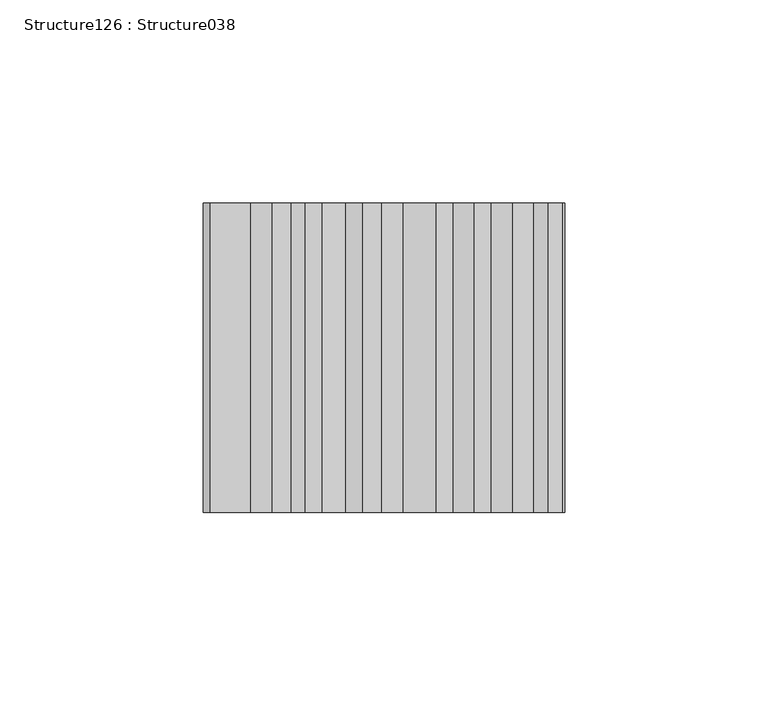
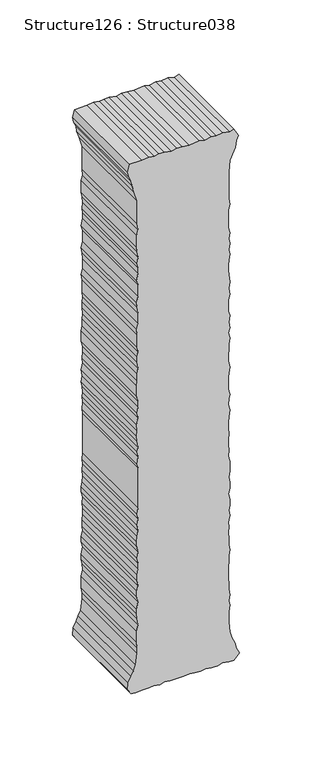
"""IFC4 building model written with IfcOpenShell, lengths in millimetres: proxy geometry, Structure126 : Structure038."""

from ifc_helpers import new_model, si_unit, frame, origin, place, context, project, spatial, polyline, outline, extrude, source, transform, mapped, element, save


def structure126_structure038_b74b1f63(model_context):
    return source(origin(), model_context, "Body", "SweptSolid", [
        extrude(outline(polyline([(3575.6853037, -44646.6654182), (3583.8864372, -44647.2591219), (3592.6700423, -44647.2591219), (3598.5284533, -44646.6654182), (3602.0280957, -44647.2591219), (3606.7295868, -44646.6654182), (3611.4134274, -44647.2591219), (3617.2718384, -44647.2591219), (3620.7971545, -44647.8415933), (3631.3410106, -44647.8415933), (3634.856699, -44647.2591219), (3640.114988, -44647.2591219), (3644.8245022, -44646.6654182), (3648.9258713, -44647.2591219), (3654.7842823, -44647.2591219), (3659.4584952, -44647.8415933), (3664.1423357, -44647.2591219), (3668.2437048, -44647.8415933), (3673.5276674, -44646.6654182), (3678.2018803, -44647.2591219), (3682.3289231, -44646.6654182), (3687.0127636, -44646.6654182), (3692.2710525, -44647.8415933), (3696.3884676, -44646.6654182), (3701.6547796, -44646.6654182), (3705.7545441, -44647.2591219), (3711.0304837, -44646.6654182), (3719.2316172, -44646.6654182), (3723.9154578, -44647.8415933), (3728.5992983, -44647.2591219), (3733.2991849, -44647.8415933), (3737.9750024, -44647.8415933), (3742.6748889, -44647.2591219), (3747.3587295, -44647.8415933), (3752.04257, -44647.8415933), (3756.7440611, -44647.2591219), (3762.5848215, -44646.6654182), (3767.2590344, -44647.8415933), (3771.9605256, -44647.2591219), (3775.4874463, -44646.6654182), (3780.1616592, -44647.8415933), (3790.7039107, -44647.8415933), (3798.9050443, -44646.6654182), (3804.1890069, -44647.8415933), (3808.8888934, -44647.8415933), (3813.5743386, -44647.2591219), (3817.6741031, -44647.2591219), (3822.932392, -44646.6654182), (3827.6162325, -44647.8415933), (3831.732043, -44646.6654182), (3836.4174882, -44647.2591219), (3842.2758992, -44646.6654182), (3845.8012153, -44647.8415933), (3855.7353217, -44647.8415933), (3859.8591552, -44646.6654182), (3865.1190488, -44647.2591219), (3870.4030114, -44646.6654182), (3879.7610648, -44647.8415933), (3884.4609514, -44647.8415933), (3888.5623205, -44647.2591219), (3893.246161, -44646.6654182), (3897.3475301, -44647.2591219), (3902.6314927, -44646.6654182), (3906.7328618, -44647.2591219), (3911.4054701, -44646.6654182), (3916.0909152, -44647.8415933), (3931.3346579, -44647.8415933), (3935.4328178, -44646.6654182), (3940.718385, -44647.2591219), (3962.9774586, -44647.2591219), (3972.3627903, -44646.6654182), (3981.7208437, -44641.9928099), (3987.5792547, -44641.3991063), (3991.0788971, -44639.6404597), (3997.5486624, -44643.1481252), (3996.390138, -44646.6654182), (3997.5486624, -44651.9413578), (3996.9645864, -44657.218902), (3997.5486624, -44661.3170619), (3996.390138, -44666.5946061), (3997.5486624, -44670.6943705), (3996.390138, -44678.9019225), (3996.9645864, -44684.1682345), (3997.5486624, -44688.8617026), (3996.390138, -44692.9630717), (3997.5486624, -44698.8134597), (3997.5486624, -44702.9196426), (3996.9645864, -44706.4305173), (3997.5486624, -44711.1223808), (3996.9645864, -44716.3967158), (3996.9645864, -44726.3564959), (3991.0788971, -44728.1151424), (3986.4046842, -44726.948595), (3982.3225704, -44725.1819254), (3978.2035506, -44724.607477), (3972.3627903, -44722.8392028), (3964.1343784, -44720.4980849), (3944.8165449, -44720.4980849), (3939.5325823, -44719.9140089), (3935.4328178, -44721.0821609), (3925.4746423, -44721.0821609), (3921.3748778, -44720.4980849), (3916.6653636, -44719.9140089), (3911.4054701, -44720.4980849), (3907.888177, -44719.9140089), (3903.2059411, -44719.9140089), (3897.3475301, -44721.0821609), (3893.246161, -44719.9140089), (3883.8881076, -44719.9140089), (3878.5784713, -44721.0821609), (3874.5043805, -44720.4980849), (3869.2444869, -44719.9140089), (3861.0192843, -44719.9140089), (3856.3161885, -44721.0821609), (3851.6612309, -44720.4980849), (3841.0900965, -44720.4980849), (3836.9919366, -44719.9140089), (3832.8921721, -44720.4980849), (3828.2163546, -44720.4980849), (3822.932392, -44719.9140089), (3818.8310229, -44720.4980849), (3812.9726119, -44720.4980849), (3808.8888934, -44721.0821609), (3800.0876378, -44721.0821609), (3795.4037973, -44719.9140089), (3790.7039107, -44719.9140089), (3785.4456218, -44720.4980849), (3781.3282066, -44719.9140089), (3776.0618947, -44721.0821609), (3770.8036057, -44720.4980849), (3766.1021146, -44721.0821609), (3762.0023501, -44720.4980849), (3756.7440611, -44719.9140089), (3753.2171405, -44720.4980849), (3748.5429276, -44719.9140089), (3742.6748889, -44720.4980849), (3739.1592005, -44719.9140089), (3705.7545441, -44719.9140089), (3700.4705815, -44720.4980849), (3696.3884676, -44719.9140089), (3691.0868544, -44720.4980849), (3686.4030139, -44719.9140089), (3681.7271964, -44720.4980849), (3677.6274319, -44721.0821609), (3673.5276674, -44721.0821609), (3668.8261762, -44719.9140089), (3663.5598643, -44720.4980849), (3658.8840468, -44719.9140089), (3654.1841602, -44719.9140089), (3649.5003197, -44720.4980849), (3644.2420307, -44720.4980849), (3640.114988, -44719.9140089), (3636.0408972, -44721.0821609), (3631.3410106, -44721.0821609), (3626.6571701, -44719.9140089), (3620.7971545, -44721.0821609), (3616.69739, -44721.0821609), (3612.5976255, -44720.4980849), (3607.3393366, -44719.9140089), (3602.0280957, -44721.0821609), (3592.6700423, -44721.0821609), (3587.9685511, -44720.4980849), (3583.2863152, -44720.4980849), (3573.9266571, -44721.6646324), (3569.8268927, -44723.4329065), (3565.7094775, -44725.1819254), (3561.025637, -44727.5310664), (3555.1848766, -44728.1151424), (3551.0658569, -44725.1819254), (3550.4833855, -44721.6646324), (3551.0658569, -44716.9904195), (3551.0658569, -44711.1223808), (3551.6675836, -44707.6050878), (3550.4833855, -44702.3291482), (3551.6675836, -44698.8134597), (3551.0658569, -44694.1376422), (3551.0658569, -44683.57774), (3551.6675836, -44678.9019225), (3551.0658569, -44674.7925304), (3550.4833855, -44670.1102945), (3551.0658569, -44666.0009024), (3550.4833855, -44661.3170619), (3550.4833855, -44656.0507499), (3551.6675836, -44652.5334569), (3550.4833855, -44647.2591219), (3550.4833855, -44643.1481252), (3555.1848766, -44639.0483607), (3559.8671125, -44641.3991063), (3565.1254015, -44642.5656537), (3569.8268927, -44644.9163993), (3575.6853037, -44646.6654182)])), frame((0.0, 247945.1599557, 0.0), z_axis=(0.0, 1.0, 0.0), x_axis=(0.0, 0.0, 1.0)), (0.0, 0.0, 1.0), 76.2),
    ])


if __name__ == "__main__":
    model = new_model("IFC4")
    model_context = context("Model", 3, world=origin())
    ifc_project = project(units=[si_unit("LENGTHUNIT", "METRE", prefix="MILLI")], contexts=[model_context])
    site = spatial("IfcSite", under=ifc_project)
    building = spatial("IfcBuilding", under=site)
    placement = place(None, origin())
    structure126_structure038_shape = structure126_structure038_b74b1f63(model_context)
    element("IfcBuildingElementProxy", 1, Name="Structure126 : Structure038", ObjectType="Structure126 : Structure038", at=placement, inside=building, context=model_context, shape_type="MappedRepresentation", body=[
        mapped(structure126_structure038_shape, transform((0.0, 0.0, 0.0), x_axis=(1.0, 0.0, 0.0), y_axis=(0.0, 1.0, 0.0), z_axis=(0.0, 0.0, 1.0))),
    ])
    save(model, "model.ifc")

# Revit data of these elements
# Type "Structure126 : Structure038"
#   NameOverride = "Structure038"
# Element 1 (IfcBuildingElementProxy, "Structure126 : Structure038")
#   Materials on its faces: "BRUSHED ALUM. LETTERING"
# Materials
#   "BRUSHED ALUM. LETTERING": class "Unassigned", colour RGB 169 181 186, transparency 0, Cost = 0
